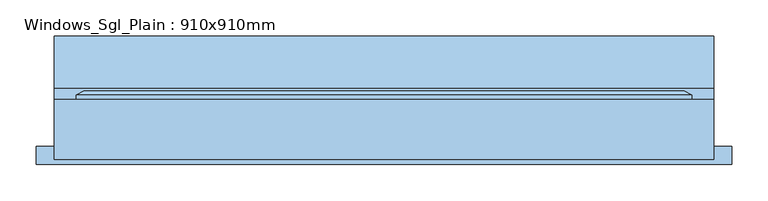
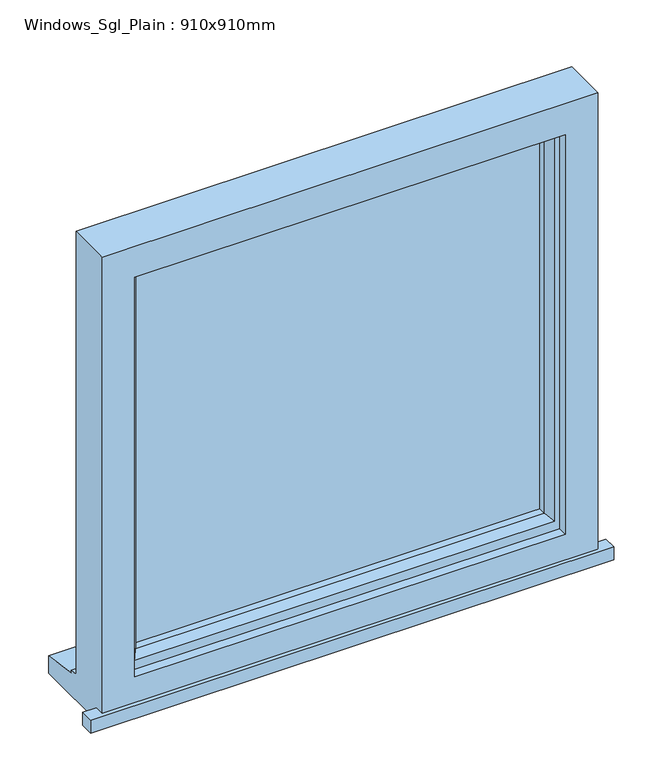
"""IFC4 building model written with IfcOpenShell, lengths in millimetres: window geometry, Windows_Sgl_Plain : 910x910mm."""

from ifc_helpers import new_model, si_unit, frame, origin, place, context, project, spatial, polyline, outline, extrude, faceted_brep, source, transform, mapped, element, save


def windows_sgl_plain_910x910mm_3bd624a2(model_context):
    return source(origin(), model_context, "Body", "SolidModel", [
        extrude(outline(polyline([(-480.0, -74.0434322), (-480.0, -49.0434322), (-455.0, -49.0434322), (-455.0, -67.0434322), (455.0, -67.0434322), (455.0, -49.0434322), (480.0, -49.0434322), (480.0, -74.0434322), (-480.0, -74.0434322)])), frame((0.0, 0.0, 1200.0), z_axis=(0.0, 0.0, 1.0), x_axis=(1.0, 0.0, 0.0)), (0.0, 0.0, 1.0), 25.0),
        faceted_brep([(-455.0, -67.0434322, 1200.0), (455.0, -67.0434322, 1200.0), (455.0, -67.0434322, 2110.0), (-455.0, -67.0434322, 2110.0), (-395.0, -67.0434322, 2050.0), (395.0, -67.0434322, 2050.0), (395.0, -67.0434322, 1275.0), (-395.0, -67.0434322, 1275.0), (-455.0, 15.9565678, 2110.0), (-455.0, 15.9565678, 1251.0), (-455.0, 30.9565678, 1249.68767), (-455.0, 30.9565678, 1244.7449676), (-455.0, 103.4565678, 1233.8088847), (-455.0, 103.4565678, 1200.0), (455.0, 15.9565678, 2110.0), (455.0, 15.9565678, 1251.0), (-415.0, 15.9565678, 2070.0), (-415.0, 15.9565678, 1263.0), (415.0, 15.9565678, 1263.0), (415.0, 15.9565678, 2070.0), (-415.0, -49.0434322, 2070.0), (-415.0, -49.0434322, 1263.0), (415.0, -49.0434322, 2070.0), (415.0, -49.0434322, 1263.0), (-395.0, -49.0434322, 2050.0), (-395.0, -49.0434322, 1275.0), (395.0, -49.0434322, 1275.0), (395.0, -49.0434322, 2050.0), (455.0, 103.4565678, 1200.0), (455.0, 103.4565678, 1233.8088847), (455.0, 30.9565678, 1244.7449676), (455.0, 30.9565678, 1249.68767)], [[[0, 1, 2, 3], [4, 5, 6, 7]], [[0, 3, 8, 9, 10, 11, 12, 13]], [[9, 8, 14, 15], [16, 17, 18, 19]], [[17, 16, 20, 21]], [[20, 22, 23, 21], [24, 25, 26, 27]], [[24, 4, 7, 25]], [[3, 2, 14, 8]], [[16, 19, 22, 20]], [[5, 4, 24, 27]], [[15, 14, 2, 1, 28, 29, 30, 31]], [[19, 18, 23, 22]], [[5, 27, 26, 6]], [[28, 1, 0, 13]], [[29, 28, 13, 12]], [[30, 29, 12, 11]], [[31, 30, 11, 10]], [[15, 31, 10, 9]], [[21, 23, 18, 17]], [[7, 6, 26, 25]]]),
        extrude(outline(polyline([(385.0, -20.0434322), (-385.0, -20.0434322), (-385.0, 3.9565678), (385.0, 3.9565678), (385.0, -20.0434322)])), frame((0.0, 0.0, 1293.0), z_axis=(0.0, 0.0, 1.0), x_axis=(1.0, 0.0, 0.0)), (0.0, 0.0, 1.0), 747.0),
        faceted_brep([(-425.0, 15.9565678, 2080.0), (-425.0, 21.7300705, 2080.0), (-425.0, 21.7300705, 1253.0), (-425.0, 15.9565678, 1253.0), (-415.0, -49.0434322, 2070.0), (-415.0, 15.9565678, 2070.0), (-415.0, 15.9565678, 1263.0), (-415.0, -49.0434322, 1263.0), (-375.0, -34.5505323, 2030.0), (-385.1480377, -49.0434322, 2040.1480377), (-385.1480377, -49.0434322, 1292.8519623), (-375.0, -34.5505323, 1303.0), (-375.0, -20.0434322, 2030.0), (-375.0, -20.0434322, 1303.0), (-385.0, 3.9565678, 2040.0), (-385.0, -20.0434322, 2040.0), (-385.0, -20.0434322, 1293.0), (-385.0, 3.9565678, 1293.0), (-375.0, 21.7300705, 2030.0), (-375.0, 3.9565678, 2030.0), (-375.0, 3.9565678, 1303.0), (-375.0, 21.7300705, 1303.0), (-392.4457548, 27.5035732, 2047.4457548), (-392.4457548, 27.5035732, 1285.5542452), (-414.2153903, 27.5035732, 2069.2153903), (-414.2153903, 27.5035732, 1263.7846097), (425.0, 21.7300705, 1253.0), (425.0, 15.9565678, 1253.0), (415.0, 15.9565678, 1263.0), (415.0, -49.0434322, 1263.0), (385.1480377, -49.0434322, 1292.8519623), (375.0, -34.5505323, 1303.0), (375.0, -20.0434322, 1303.0), (385.0, -20.0434322, 1293.0), (385.0, 3.9565678, 1293.0), (375.0, 3.9565678, 1303.0), (375.0, 21.7300705, 1303.0), (392.4457548, 27.5035732, 1285.5542452), (414.2153903, 27.5035732, 1263.7846097), (425.0, 21.7300705, 2080.0), (425.0, 15.9565678, 2080.0), (415.0, 15.9565678, 2070.0), (415.0, -49.0434322, 2070.0), (385.1480377, -49.0434322, 2040.1480377), (375.0, -34.5505323, 2030.0), (375.0, -20.0434322, 2030.0), (385.0, -20.0434322, 2040.0), (385.0, 3.9565678, 2040.0), (375.0, 3.9565678, 2030.0), (375.0, 21.7300705, 2030.0), (392.4457548, 27.5035732, 2047.4457548), (414.2153903, 27.5035732, 2069.2153903)], [[[0, 1, 2, 3]], [[4, 5, 6, 7]], [[8, 9, 10, 11]], [[12, 8, 11, 13]], [[14, 15, 16, 17]], [[18, 19, 20, 21]], [[22, 18, 21, 23]], [[1, 24, 25, 2]], [[3, 2, 26, 27]], [[7, 6, 28, 29]], [[11, 10, 30, 31]], [[13, 11, 31, 32]], [[17, 16, 33, 34]], [[21, 20, 35, 36]], [[23, 21, 36, 37]], [[2, 25, 38, 26]], [[27, 26, 39, 40]], [[29, 28, 41, 42]], [[31, 30, 43, 44]], [[32, 31, 44, 45]], [[34, 33, 46, 47]], [[36, 35, 48, 49]], [[37, 36, 49, 50]], [[26, 38, 51, 39]], [[40, 39, 1, 0]], [[3, 27, 40, 0], [5, 41, 28, 6]], [[42, 41, 5, 4]], [[7, 29, 42, 4], [9, 43, 30, 10]], [[44, 43, 9, 8]], [[45, 44, 8, 12]], [[15, 46, 33, 16], [13, 32, 45, 12]], [[47, 46, 15, 14]], [[17, 34, 47, 14], [19, 48, 35, 20]], [[49, 48, 19, 18]], [[50, 49, 18, 22]], [[24, 51, 38, 25], [23, 37, 50, 22]], [[39, 51, 24, 1]]]),
    ])


if __name__ == "__main__":
    model = new_model("IFC4")
    model_context = context("Model", 3, world=origin())
    ifc_project = project(units=[si_unit("LENGTHUNIT", "METRE", prefix="MILLI")], contexts=[model_context])
    site = spatial("IfcSite", under=ifc_project)
    building = spatial("IfcBuilding", under=site)
    placement = place(None, origin())
    windows_sgl_plain_910x910mm_shape = windows_sgl_plain_910x910mm_3bd624a2(model_context)
    element("IfcWindow", 1, ObjectType="Windows_Sgl_Plain : 910x910mm", at=placement, inside=building, context=model_context, shape_type="MappedRepresentation", body=[
        mapped(windows_sgl_plain_910x910mm_shape, transform((0.0, 0.0, 0.0), x_axis=(1.0, 0.0, 0.0), y_axis=(0.0, 1.0, 0.0), z_axis=(0.0, 0.0, 1.0))),
    ])
    save(model, "model.ifc")

# Revit data of these elements
# Type "Windows_Sgl_Plain : 910x910mm"
#   Type Mark = "44"
#   Operation = "SinglePanel"
#   Construction Type Id = "SGL"
#   Manufacturer = "Revit"
#   Keynote = "L10"
#   Analytic Construction = "Large single-glazed windows"
#   Wrap Layers (Ext) from Ext = 102.5 mm
#   Wrap Layers (Int) from Ext = 177.5 mm
#   Window Board Projection = 25 mm
#   Window Board Extension = 25 mm
#   Visual Light Transmittance = 0.9
#   Solar Heat Gain Coefficient = 0.86
#   Rough Width = 910 mm
#   Rough Height = 910 mm
#   Height = 910 mm
#   Width = 910 mm
#   Heat Transfer Coefficient (U) = 5.5617 W/(m²·K)
#   Glazing Thickness = 24 mm
#   FrameOffset - External = 50 mm
#   Frame Depth = 65 mm
#   Default Head Height = 2110 mm
#   Cill Depth = 87.5 mm
#   Cavity Closer Width = 50 mm
#   Cavity Closer Offset from Ext = 102.5 mm
#   Cavity Closer Depth = 85 mm
#   Define Thermal Properties by = 1
#   Vis - Cavity Closers = yes
#   Define Thermal Properties by = 1
#   Material Trim = Window Frame
#   Material Glass = Glass
#   Material Frame = Window Frame
#   Wall Closure = (empty or 0)
# Element 1 (IfcWindow, "Windows_Sgl_Plain : 910x910mm")
#   Materials on its faces: "Window Frame", "Glass"
# Materials
#   "Window Frame": class "Miscellaneous", colour RGB 249 249 249, transparency 0, Keynote = "L10", Cost = 0
#   "Glass": class "Glass", colour RGB 0 128 192, transparency 0.9, Description = "Soda Lime Glass", Cost = 0
